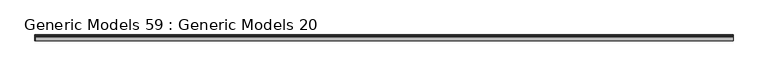
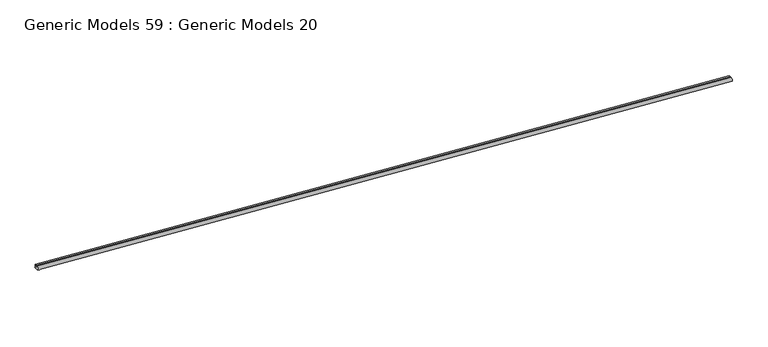
"""IFC4 building model written with IfcOpenShell, lengths in millimetres: proxy geometry, Generic Models 59 : Generic Models 20."""

import ifcopenshell
import ifcopenshell.guid

model = None  # the IFC model being written
_history = None  # IfcOwnerHistory: only IFC2X3 demands one
_inside = {}  # id of a spatial element -> (the spatial element, [elements in it])
_under = {}  # id of a project, library or spatial element -> (it, [spatial elements below it])
_declared = {}  # id of a project -> (the project, [libraries it declares])
_typed = {}  # id of a type object -> (the type object, [elements of that type])
_made_of = {}  # id of a material, layer set ... -> (it, [elements and type objects made of it])


def new_model(schema):
    """Start an empty IFC model of exactly this schema.

    Asked for "IFC4X3", IfcOpenShell would pick the latest addendum, in which some entities
    have other attributes; the version numbers below select the first issue.
    IFC2X3 requires an IfcOwnerHistory on every rooted entity: one is made here for all.
    """
    global model, _history
    if schema == "IFC4X3":
        model = ifcopenshell.file(schema_version=(4, 3, 0, 0))
    else:
        model = ifcopenshell.file(schema=schema)
    _inside.clear()
    _under.clear()
    _declared.clear()
    _typed.clear()
    _made_of.clear()
    _history = None
    if model.schema == "IFC2X3":
        org = make("IfcOrganization", Name="unknown")
        user = make(
            "IfcPersonAndOrganization",
            ThePerson=make("IfcPerson", FamilyName="unknown"),
            TheOrganization=org,
        )
        app = make(
            "IfcApplication",
            ApplicationDeveloper=org,
            Version="unknown",
            ApplicationFullName="unknown",
            ApplicationIdentifier="unknown",
        )
        _history = make(
            "IfcOwnerHistory",
            OwningUser=user,
            OwningApplication=app,
            ChangeAction="ADDED",
            CreationDate=0,
        )
    return model


def make(cls, **values):
    """One entity of the class cls with the attributes given. An attribute that is None is left unset."""
    return model.create_entity(
        cls, **{name: value for name, value in values.items() if value is not None}
    )


def rooted(cls, **values):
    """An entity with a GlobalId (a new one), such as an element, a storey or a relation."""
    return make(cls, GlobalId=ifcopenshell.guid.new(), OwnerHistory=_history, **values)


def si_unit(unit_type, name, prefix=None):
    """IfcSIUnit, for example si_unit("LENGTHUNIT", "METRE", prefix="MILLI")."""
    return make("IfcSIUnit", UnitType=unit_type, Prefix=prefix, Name=name)


def assignment(units):
    """IfcUnitAssignment: the units of a project."""
    return None if units is None else make("IfcUnitAssignment", Units=units)


def point(xyz):
    """IfcCartesianPoint."""
    return None if xyz is None else make("IfcCartesianPoint", Coordinates=xyz)


def direction(xyz):
    """IfcDirection."""
    return None if xyz is None else make("IfcDirection", DirectionRatios=xyz)


def frame(location, z_axis=None, x_axis=None):
    """IfcAxis2Placement3D, a coordinate frame: its origin and axes. An axis left out is left unset."""
    return make(
        "IfcAxis2Placement3D",
        Location=point(location),
        Axis=direction(z_axis),
        RefDirection=direction(x_axis),
    )


def origin():
    """The frame at (0, 0, 0) with its axes left unset."""
    return frame((0.0, 0.0, 0.0))


def place(relative_to, where):
    """IfcLocalPlacement: puts the frame where relative to a parent placement (None: the world)."""
    return make(
        "IfcLocalPlacement", PlacementRelTo=relative_to, RelativePlacement=where
    )


def context(
    kind, dimensions, precision=None, world=None, true_north=None, identifier=None
):
    """IfcGeometricRepresentationContext, for example the 3D "Model" context."""
    return make(
        "IfcGeometricRepresentationContext",
        ContextIdentifier=identifier,
        ContextType=kind,
        CoordinateSpaceDimension=dimensions,
        Precision=precision,
        WorldCoordinateSystem=world,
        TrueNorth=true_north,
    )


def project(units=None, contexts=None):
    """IfcProject with its units and contexts."""
    return rooted(
        "IfcProject",
        Name="project",
        RepresentationContexts=contexts,
        UnitsInContext=assignment(units),
    )


def spatial(cls, under=None, at=None, **own):
    """A site, building, storey or space (cls), placed at a placement, below another one or the project."""
    s = rooted(cls, ObjectPlacement=at, **own)
    if under is not None:
        _under.setdefault(under.id(), (under, []))[1].append(s)
    return s


def polyline(points):
    """IfcPolyline through the points."""
    return make("IfcPolyline", Points=[point(p) for p in points])


def circle_curve(where, radius):
    """IfcCircle in the frame where."""
    return make("IfcCircle", Position=where, Radius=radius)


def ellipse_curve(where, semi_axis1, semi_axis2):
    """IfcEllipse in the frame where."""
    return make(
        "IfcEllipse", Position=where, SemiAxis1=semi_axis1, SemiAxis2=semi_axis2
    )


def trimmed(basis, trim1, trim2, sense, master):
    """IfcTrimmedCurve: the piece of a basis curve between two trims."""
    return make(
        "IfcTrimmedCurve",
        BasisCurve=basis,
        Trim1=trim1,
        Trim2=trim2,
        SenseAgreement=sense,
        MasterRepresentation=master,
    )


def shape(context_of_items, identifier, shape_type, items):
    """IfcShapeRepresentation: the items that make up one representation, for example the "Body"."""
    return make(
        "IfcShapeRepresentation",
        ContextOfItems=context_of_items,
        RepresentationIdentifier=identifier,
        RepresentationType=shape_type,
        Items=items,
    )


def source(mapping_origin, context_of_items, identifier, shape_type, items):
    """IfcRepresentationMap: a shape defined once, which mapped items show again and again."""
    return make(
        "IfcRepresentationMap",
        MappingOrigin=mapping_origin,
        MappedRepresentation=shape(context_of_items, identifier, shape_type, items),
    )


def transform(
    local_origin,
    x_axis=None,
    y_axis=None,
    z_axis=None,
    scale=None,
    scale2=None,
    scale3=None,
    uniform=True,
):
    """IfcCartesianTransformationOperator3D, or its non-uniform kind. x_axis, y_axis, z_axis: its Axis1, 2, 3."""
    if uniform:
        return make(
            "IfcCartesianTransformationOperator3D",
            Axis1=direction(x_axis),
            Axis2=direction(y_axis),
            LocalOrigin=point(local_origin),
            Scale=scale,
            Axis3=direction(z_axis),
        )
    return make(
        "IfcCartesianTransformationOperator3DnonUniform",
        Axis1=direction(x_axis),
        Axis2=direction(y_axis),
        LocalOrigin=point(local_origin),
        Scale=scale,
        Axis3=direction(z_axis),
        Scale2=scale2,
        Scale3=scale3,
    )


def mapped(mapping_source, mapping_target):
    """IfcMappedItem: shows the shape of a source again, moved by a transform."""
    return make(
        "IfcMappedItem", MappingSource=mapping_source, MappingTarget=mapping_target
    )


def made_of(thing, what):
    """Note that an element or type object is made of a material, layer set ...; save() writes the relation."""
    if what is not None:
        _made_of.setdefault(what.id(), (what, []))[1].append(thing)
    return thing


def element(
    cls,
    number,
    at=None,
    inside=None,
    cuts=None,
    type_object=None,
    material=None,
    context=None,
    identifier="Body",
    shape_type=None,
    held_by="IfcProductDefinitionShape",
    body=None,
    shapes=None,
    **own,
):
    """One element of the class cls, such as IfcWall. Its Tag is "e" and its number.

    at: its placement. inside: the storey or other place that contains it. cuts: it is an
    opening in that element (IfcRelVoidsElement). A single representation is given by context,
    identifier, shape_type and body (its items); several are given by shapes. held_by: the class
    of the entity that holds the representations. save() writes the other relations.
    """
    e = rooted(cls, Tag="e%d" % number, ObjectPlacement=at, **own)
    if body is not None:
        shapes = [shape(context, identifier, shape_type, body)]
    if shapes is not None:
        e.Representation = make(held_by, Representations=shapes)
    if inside is not None:
        _inside.setdefault(inside.id(), (inside, []))[1].append(e)
    if cuts is not None:
        rooted(
            "IfcRelVoidsElement", RelatingBuildingElement=cuts, RelatedOpeningElement=e
        )
    if type_object is not None:
        _typed.setdefault(type_object.id(), (type_object, []))[1].append(e)
    return made_of(e, material)


def aggregate(whole, parts):
    """IfcRelAggregates: a whole, such as a stair, and the parts it consists of."""
    return rooted("IfcRelAggregates", RelatingObject=whole, RelatedObjects=parts)


def save(model, path):
    """Write the relations noted so far, then the file.

    IfcRelAggregates (storeys below a building ...), IfcRelContainedInSpatialStructure (elements
    in a storey), IfcRelDefinesByType, IfcRelAssociatesMaterial and IfcRelDeclares: one each for
    every whole, place, type object, material and project.
    """
    for whole, parts in _under.values():
        aggregate(whole, parts)
    for where, things in _inside.values():
        rooted(
            "IfcRelContainedInSpatialStructure",
            RelatedElements=things,
            RelatingStructure=where,
        )
    for kind, things in _typed.values():
        rooted("IfcRelDefinesByType", RelatedObjects=things, RelatingType=kind)
    for what, things in _made_of.values():
        rooted("IfcRelAssociatesMaterial", RelatedObjects=things, RelatingMaterial=what)
    for by, libraries in _declared.values():
        rooted("IfcRelDeclares", RelatingContext=by, RelatedDefinitions=libraries)
    model.write(path)


def plane_surface(at):
    """IfcPlane: the flat surface through the origin of the frame at, square to its z axis."""
    return make("IfcPlane", Position=at)


def cylinder_surface(at, radius):
    """IfcCylindricalSurface: all points at the distance radius from the z axis of the frame at."""
    return make("IfcCylindricalSurface", Position=at, Radius=radius)


def revolved_surface(curve, axis_point, axis_direction):
    """IfcSurfaceOfRevolution: the curve turned about the line through axis_point along axis_direction."""
    return make(
        "IfcSurfaceOfRevolution",
        SweptCurve=make("IfcArbitraryOpenProfileDef", ProfileType="CURVE", Curve=curve),
        AxisPosition=make("IfcAxis1Placement", Location=point(axis_point), Axis=direction(axis_direction)),
    )


def extruded_surface(curve, direction_of_extrusion, depth):
    """IfcSurfaceOfLinearExtrusion: the curve pushed along a direction by depth."""
    return make(
        "IfcSurfaceOfLinearExtrusion",
        SweptCurve=make("IfcArbitraryOpenProfileDef", ProfileType="CURVE", Curve=curve),
        ExtrudedDirection=direction(direction_of_extrusion),
        Depth=depth,
    )


def advanced_brep(points, edges, surfaces, faces):
    """IfcAdvancedBrep: a solid bounded by faces that lie on surfaces and meet in shared edges.

    An edge is (start, end): straight between two places in points (the first is 0);
    or (start, end, curve); or (start, end, curve, False) where it runs against its curve.
    A face is (place in surfaces, loops), or (place, loops, False) where it looks against
    its surface's normal. A loop lists edges by number (the first is 1), with a minus sign
    where the edge is run from its end to its start. The first loop is the outer one.
    """
    corners = [point(p) for p in points]
    vertices = [make("IfcVertexPoint", VertexGeometry=c) for c in corners]
    made = []
    for start, end, *more in edges:
        made.append(
            make(
                "IfcEdgeCurve",
                EdgeStart=vertices[start],
                EdgeEnd=vertices[end],
                EdgeGeometry=more[0] if more else make("IfcPolyline", Points=[corners[start], corners[end]]),
                SameSense=more[1] if len(more) > 1 else True,
            )
        )
    hull = []
    for where, loops, *sense in faces:
        bounds = []
        for j, loop in enumerate(loops):
            ring = [make("IfcOrientedEdge", EdgeElement=made[abs(k) - 1], Orientation=k > 0) for k in loop]
            bounds.append(
                make(
                    "IfcFaceOuterBound" if j == 0 else "IfcFaceBound",
                    Bound=make("IfcEdgeLoop", EdgeList=ring),
                    Orientation=True,
                )
            )
        hull.append(make("IfcAdvancedFace", Bounds=bounds, FaceSurface=surfaces[where], SameSense=sense[0] if sense else True))
    return make("IfcAdvancedBrep", Outer=make("IfcClosedShell", CfsFaces=hull))


def generic_models_59_generic_models_20_48713198(model_context):
    return source(origin(), model_context, "Body", "AdvancedBrep", [
        advanced_brep(
        [(27444.1367123, 25554.7652073, 272206.9153252), (27444.1367123, 25551.5902073, 272206.9153252), (27444.2159739, 25550.638448, 272208.1835092), (27444.4535532, 25550.638448, 272211.984775), (27444.5328147, 25551.5902073, 272213.252959), (27444.5328147, 25554.7652073, 272213.252959), (28939.8183027, 25554.7652073, 272113.4351647), (28940.214405, 25554.7652073, 272119.7727986), (28940.214405, 25551.5902073, 272119.7727986), (28940.1351435, 25550.638448, 272118.5046145), (28939.8975642, 25550.638448, 272114.7033488), (28939.8183027, 25551.5902073, 272113.4351647)],
        [
            (0, 1),
            (1, 2, circle_curve(frame((27444.3347635, 25554.5049478, 272210.0841421), z_axis=(-0.9980525759468363, 0.0, 0.0623783267320061), x_axis=(-0.0623783267320061, 0.0, -0.9980525759468363)), 4.3100275)),
            (2, 3, ellipse_curve(frame((27444.3347635, 25546.8277073, 272210.0841421), z_axis=(-0.9980525759468363, 0.0, 0.0623783267320061), x_axis=(0.0, 1.0, 0.0)), 4.7625, 3.175)),
            (3, 4, circle_curve(frame((27444.3347635, 25554.5049478, 272210.0841421), z_axis=(-0.9980525759468363, 0.0, 0.0623783267320061), x_axis=(-0.0623783267320061, 0.0, -0.9980525759468363)), 4.3100275)),
            (4, 5),
            (5, 0, circle_curve(frame((27444.3347635, 25557.6799478, 272210.0841421), z_axis=(0.9980525759468363, 0.0, -0.0623783267320061), x_axis=(-0.0623783267320061, 0.0, -0.9980525759468363)), 4.3100275)),
            (6, 7, circle_curve(frame((28940.0163538, 25557.6799478, 272116.6039817), z_axis=(-0.9980525759468363, 0.0, 0.0623783267320061), x_axis=(-0.0623783267320061, 0.0, -0.9980525759468363)), 4.3100275)),
            (7, 8),
            (8, 9, circle_curve(frame((28940.0163538, 25554.5049478, 272116.6039817), z_axis=(0.9980525759468363, 0.0, -0.0623783267320061), x_axis=(-0.0623783267320061, 0.0, -0.9980525759468363)), 4.3100275)),
            (9, 10, ellipse_curve(frame((28940.0163538, 25546.8277073, 272116.6039817), z_axis=(0.9980525759468363, 0.0, -0.0623783267320061), x_axis=(0.0, 1.0, 0.0)), 4.7625, 3.175)),
            (10, 11, circle_curve(frame((28940.0163538, 25554.5049478, 272116.6039817), z_axis=(0.9980525759468363, 0.0, -0.0623783267320061), x_axis=(-0.0623783267320061, 0.0, -0.9980525759468363)), 4.3100275)),
            (11, 6),
            (0, 6),
            (11, 1),
            (5, 7),
            (4, 8),
            (3, 9),
            (2, 10),
        ],
        [
            plane_surface(frame((27444.5328147, 25554.7652073, 272213.252959), z_axis=(-0.9980525759468363, 0.0, 0.0623783267320061), x_axis=(0.0, 1.0, 0.0))),
            plane_surface(frame((28940.214405, 25554.7652073, 272119.7727986), z_axis=(0.9980525759468363, 0.0, -0.0623783267320061), x_axis=(0.0, 1.0, 0.0))),
            plane_surface(frame((27444.1367123, 25554.7652073, 272206.9153252), z_axis=(-0.06237832673200577, 0.0, -0.9980525759468362), x_axis=(0.9980525759468362, 0.0, -0.06237832673200577))),
            revolved_surface(polyline([(28939.74750158539, 25557.6799478, 272112.302347606), (27444.065911182024, 25557.6799478, 272205.7825080521)]), (27444.3347635, 25557.6799478, 272210.0841421), (0.9980525759468363, 0.0, -0.0623783267320061)),
            plane_surface(frame((27444.5328147, 25551.5902073, 272213.252959), z_axis=(0.06237832673200577, 0.0, 0.9980525759468362), x_axis=(0.9980525759468362, 0.0, -0.06237832673200577))),
            cylinder_surface(frame((27444.3347635, 25554.5049478, 272210.0841421), z_axis=(-0.9980525759468363, 0.0, 0.0623783267320061), x_axis=(-0.0623783267320061, 0.0, -0.9980525759468363)), 4.3100275),
            extruded_surface(trimmed(ellipse_curve(frame((28940.0163538, 25546.8277073, 272116.6039817), z_axis=(-0.9980525759468363, 0.0, 0.0623783267320061), x_axis=(0.0, 1.0, 0.0)), 4.7625, 3.175), [point((28939.8975642, 25550.638448, 272114.7033488))], [point((28940.1351435, 25550.638448, 272118.5046145))], True, "CARTESIAN"), (-1495.6815903000024, 0.0, 93.48016039998038), 1498.5999999835683),
        ],
        [
            (0, [[1, 2, 3, 4, 5, 6]]),
            (1, [[7, 8, 9, 10, 11, 12]]),
            (2, [[-1, 13, -12, 14]]),
            (3, [[-6, 15, -7, -13]]),
            (4, [[-5, 16, -8, -15]]),
            (5, [[-4, 17, -9, -16]]),
            (6, [[-3, 18, -10, -17]]),
            (5, [[-2, -14, -11, -18]]),
        ],
    ),
    ])


if __name__ == "__main__":
    model = new_model("IFC4")
    model_context = context("Model", 3, world=origin())
    ifc_project = project(units=[si_unit("LENGTHUNIT", "METRE", prefix="MILLI")], contexts=[model_context])
    site = spatial("IfcSite", under=ifc_project)
    building = spatial("IfcBuilding", under=site)
    placement = place(None, origin())
    generic_models_59_generic_models_20_shape = generic_models_59_generic_models_20_48713198(model_context)
    element("IfcBuildingElementProxy", 1, Name="Generic Models 59 : Generic Models 20", ObjectType="Generic Models 59 : Generic Models 20", at=placement, inside=building, context=model_context, shape_type="MappedRepresentation", body=[
        mapped(generic_models_59_generic_models_20_shape, transform((0.0, 0.0, 0.0), x_axis=(1.0, 0.0, 0.0), y_axis=(0.0, 1.0, 0.0), z_axis=(0.0, 0.0, 1.0))),
    ])
    save(model, "model.ifc")

# Revit data of these elements
# Element 1 (IfcBuildingElementProxy, "Generic Models 59 : Generic Models 20")
#   Materials on its faces: "SEALANT (& BACKER ROD IF NECESSARY)"
# Materials
#   "SEALANT (& BACKER ROD IF NECESSARY)": class "Generic", colour RGB 176 213 108, transparency 0, Cost = 0
